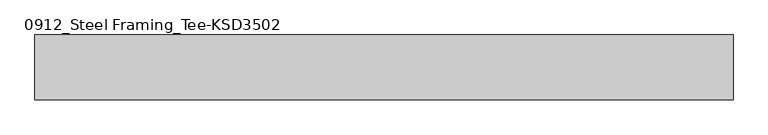
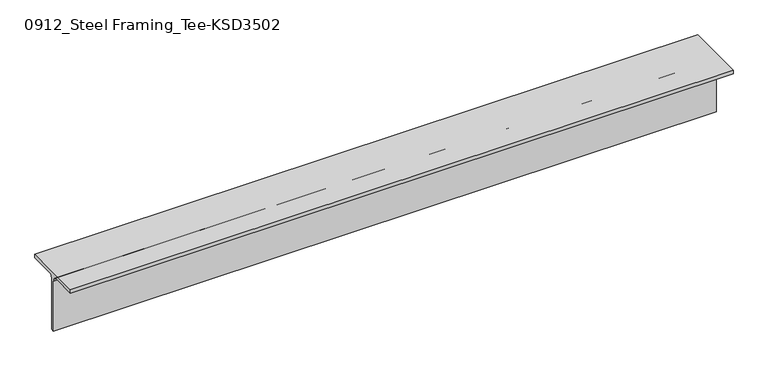
"""IFC4 building model written with IfcOpenShell, lengths in millimetres: member geometry, 0912_Steel Framing_Tee-KSD3502 : H_SB_ASB_CT-150x150x6.5x9."""

import ifcopenshell
import ifcopenshell.guid

model = None  # the IFC model being written
_history = None  # IfcOwnerHistory: only IFC2X3 demands one
_inside = {}  # id of a spatial element -> (the spatial element, [elements in it])
_under = {}  # id of a project, library or spatial element -> (it, [spatial elements below it])
_declared = {}  # id of a project -> (the project, [libraries it declares])
_typed = {}  # id of a type object -> (the type object, [elements of that type])
_made_of = {}  # id of a material, layer set ... -> (it, [elements and type objects made of it])


def new_model(schema):
    """Start an empty IFC model of exactly this schema.

    Asked for "IFC4X3", IfcOpenShell would pick the latest addendum, in which some entities
    have other attributes; the version numbers below select the first issue.
    IFC2X3 requires an IfcOwnerHistory on every rooted entity: one is made here for all.
    """
    global model, _history
    if schema == "IFC4X3":
        model = ifcopenshell.file(schema_version=(4, 3, 0, 0))
    else:
        model = ifcopenshell.file(schema=schema)
    _inside.clear()
    _under.clear()
    _declared.clear()
    _typed.clear()
    _made_of.clear()
    _history = None
    if model.schema == "IFC2X3":
        org = make("IfcOrganization", Name="unknown")
        user = make(
            "IfcPersonAndOrganization",
            ThePerson=make("IfcPerson", FamilyName="unknown"),
            TheOrganization=org,
        )
        app = make(
            "IfcApplication",
            ApplicationDeveloper=org,
            Version="unknown",
            ApplicationFullName="unknown",
            ApplicationIdentifier="unknown",
        )
        _history = make(
            "IfcOwnerHistory",
            OwningUser=user,
            OwningApplication=app,
            ChangeAction="ADDED",
            CreationDate=0,
        )
    return model


def make(cls, **values):
    """One entity of the class cls with the attributes given. An attribute that is None is left unset."""
    return model.create_entity(
        cls, **{name: value for name, value in values.items() if value is not None}
    )


def rooted(cls, **values):
    """An entity with a GlobalId (a new one), such as an element, a storey or a relation."""
    return make(cls, GlobalId=ifcopenshell.guid.new(), OwnerHistory=_history, **values)


def si_unit(unit_type, name, prefix=None):
    """IfcSIUnit, for example si_unit("LENGTHUNIT", "METRE", prefix="MILLI")."""
    return make("IfcSIUnit", UnitType=unit_type, Prefix=prefix, Name=name)


def assignment(units):
    """IfcUnitAssignment: the units of a project."""
    return None if units is None else make("IfcUnitAssignment", Units=units)


def point(xyz):
    """IfcCartesianPoint."""
    return None if xyz is None else make("IfcCartesianPoint", Coordinates=xyz)


def direction(xyz):
    """IfcDirection."""
    return None if xyz is None else make("IfcDirection", DirectionRatios=xyz)


def frame(location, z_axis=None, x_axis=None):
    """IfcAxis2Placement3D, a coordinate frame: its origin and axes. An axis left out is left unset."""
    return make(
        "IfcAxis2Placement3D",
        Location=point(location),
        Axis=direction(z_axis),
        RefDirection=direction(x_axis),
    )


def frame_2d(location, x_axis=None):
    """IfcAxis2Placement2D, a coordinate frame in the plane: its origin and x axis."""
    return make(
        "IfcAxis2Placement2D", Location=point(location), RefDirection=direction(x_axis)
    )


def origin():
    """The frame at (0, 0, 0) with its axes left unset."""
    return frame((0.0, 0.0, 0.0))


def place(relative_to, where):
    """IfcLocalPlacement: puts the frame where relative to a parent placement (None: the world)."""
    return make(
        "IfcLocalPlacement", PlacementRelTo=relative_to, RelativePlacement=where
    )


def context(
    kind, dimensions, precision=None, world=None, true_north=None, identifier=None
):
    """IfcGeometricRepresentationContext, for example the 3D "Model" context."""
    return make(
        "IfcGeometricRepresentationContext",
        ContextIdentifier=identifier,
        ContextType=kind,
        CoordinateSpaceDimension=dimensions,
        Precision=precision,
        WorldCoordinateSystem=world,
        TrueNorth=true_north,
    )


def project(units=None, contexts=None):
    """IfcProject with its units and contexts."""
    return rooted(
        "IfcProject",
        Name="project",
        RepresentationContexts=contexts,
        UnitsInContext=assignment(units),
    )


def spatial(cls, under=None, at=None, **own):
    """A site, building, storey or space (cls), placed at a placement, below another one or the project."""
    s = rooted(cls, ObjectPlacement=at, **own)
    if under is not None:
        _under.setdefault(under.id(), (under, []))[1].append(s)
    return s


def polyline(points):
    """IfcPolyline through the points."""
    return make("IfcPolyline", Points=[point(p) for p in points])


def circle_curve(where, radius):
    """IfcCircle in the frame where."""
    return make("IfcCircle", Position=where, Radius=radius)


def trimmed(basis, trim1, trim2, sense, master):
    """IfcTrimmedCurve: the piece of a basis curve between two trims."""
    return make(
        "IfcTrimmedCurve",
        BasisCurve=basis,
        Trim1=trim1,
        Trim2=trim2,
        SenseAgreement=sense,
        MasterRepresentation=master,
    )


def segment(curve, same_sense, transition):
    """IfcCompositeCurveSegment."""
    return make(
        "IfcCompositeCurveSegment",
        Transition=transition,
        SameSense=same_sense,
        ParentCurve=curve,
    )


def composite_curve(segments, self_intersect=None):
    """IfcCompositeCurve: segments joined end to end."""
    return make("IfcCompositeCurve", Segments=segments, SelfIntersect=self_intersect)


def outline(outer, holes=None, kind="AREA"):
    """IfcArbitraryClosedProfileDef: a profile drawn as a closed curve; with holes, ...WithVoids."""
    if holes is None:
        return make("IfcArbitraryClosedProfileDef", ProfileType=kind, OuterCurve=outer)
    return make(
        "IfcArbitraryProfileDefWithVoids",
        ProfileType=kind,
        OuterCurve=outer,
        InnerCurves=holes,
    )


def extrude(swept, where, along, depth):
    """IfcExtrudedAreaSolid: the profile swept, set in the frame where, extruded along a direction by depth."""
    return make(
        "IfcExtrudedAreaSolid",
        SweptArea=swept,
        Position=where,
        ExtrudedDirection=direction(along),
        Depth=depth,
    )


def shape(context_of_items, identifier, shape_type, items):
    """IfcShapeRepresentation: the items that make up one representation, for example the "Body"."""
    return make(
        "IfcShapeRepresentation",
        ContextOfItems=context_of_items,
        RepresentationIdentifier=identifier,
        RepresentationType=shape_type,
        Items=items,
    )


def source(mapping_origin, context_of_items, identifier, shape_type, items):
    """IfcRepresentationMap: a shape defined once, which mapped items show again and again."""
    return make(
        "IfcRepresentationMap",
        MappingOrigin=mapping_origin,
        MappedRepresentation=shape(context_of_items, identifier, shape_type, items),
    )


def transform(
    local_origin,
    x_axis=None,
    y_axis=None,
    z_axis=None,
    scale=None,
    scale2=None,
    scale3=None,
    uniform=True,
):
    """IfcCartesianTransformationOperator3D, or its non-uniform kind. x_axis, y_axis, z_axis: its Axis1, 2, 3."""
    if uniform:
        return make(
            "IfcCartesianTransformationOperator3D",
            Axis1=direction(x_axis),
            Axis2=direction(y_axis),
            LocalOrigin=point(local_origin),
            Scale=scale,
            Axis3=direction(z_axis),
        )
    return make(
        "IfcCartesianTransformationOperator3DnonUniform",
        Axis1=direction(x_axis),
        Axis2=direction(y_axis),
        LocalOrigin=point(local_origin),
        Scale=scale,
        Axis3=direction(z_axis),
        Scale2=scale2,
        Scale3=scale3,
    )


def mapped(mapping_source, mapping_target):
    """IfcMappedItem: shows the shape of a source again, moved by a transform."""
    return make(
        "IfcMappedItem", MappingSource=mapping_source, MappingTarget=mapping_target
    )


def made_of(thing, what):
    """Note that an element or type object is made of a material, layer set ...; save() writes the relation."""
    if what is not None:
        _made_of.setdefault(what.id(), (what, []))[1].append(thing)
    return thing


def element(
    cls,
    number,
    at=None,
    inside=None,
    cuts=None,
    type_object=None,
    material=None,
    context=None,
    identifier="Body",
    shape_type=None,
    held_by="IfcProductDefinitionShape",
    body=None,
    shapes=None,
    **own,
):
    """One element of the class cls, such as IfcWall. Its Tag is "e" and its number.

    at: its placement. inside: the storey or other place that contains it. cuts: it is an
    opening in that element (IfcRelVoidsElement). A single representation is given by context,
    identifier, shape_type and body (its items); several are given by shapes. held_by: the class
    of the entity that holds the representations. save() writes the other relations.
    """
    e = rooted(cls, Tag="e%d" % number, ObjectPlacement=at, **own)
    if body is not None:
        shapes = [shape(context, identifier, shape_type, body)]
    if shapes is not None:
        e.Representation = make(held_by, Representations=shapes)
    if inside is not None:
        _inside.setdefault(inside.id(), (inside, []))[1].append(e)
    if cuts is not None:
        rooted(
            "IfcRelVoidsElement", RelatingBuildingElement=cuts, RelatedOpeningElement=e
        )
    if type_object is not None:
        _typed.setdefault(type_object.id(), (type_object, []))[1].append(e)
    return made_of(e, material)


def aggregate(whole, parts):
    """IfcRelAggregates: a whole, such as a stair, and the parts it consists of."""
    return rooted("IfcRelAggregates", RelatingObject=whole, RelatedObjects=parts)


def save(model, path):
    """Write the relations noted so far, then the file.

    IfcRelAggregates (storeys below a building ...), IfcRelContainedInSpatialStructure (elements
    in a storey), IfcRelDefinesByType, IfcRelAssociatesMaterial and IfcRelDeclares: one each for
    every whole, place, type object, material and project.
    """
    for whole, parts in _under.values():
        aggregate(whole, parts)
    for where, things in _inside.values():
        rooted(
            "IfcRelContainedInSpatialStructure",
            RelatedElements=things,
            RelatingStructure=where,
        )
    for kind, things in _typed.values():
        rooted("IfcRelDefinesByType", RelatedObjects=things, RelatingType=kind)
    for what, things in _made_of.values():
        rooted("IfcRelAssociatesMaterial", RelatedObjects=things, RelatingMaterial=what)
    for by, libraries in _declared.values():
        rooted("IfcRelDeclares", RelatingContext=by, RelatedDefinitions=libraries)
    model.write(path)


def member_0912_steel_framing_tee_ksd3502_5d1e5f2d(model_context):
    return source(origin(), model_context, "Body", "SweptSolid", [
        extrude(outline(composite_curve([segment(polyline([(-75.0, 75.0), (75.0, 75.0), (75.0, 66.0), (16.25, 66.0)]), True, "CONTINUOUS"), segment(trimmed(circle_curve(frame_2d((16.25, 53.0)), 13.0), [point((16.25, 66.0))], [point((3.25, 53.0))], True, "CARTESIAN"), True, "CONTINUOUS"), segment(polyline([(3.25, 53.0), (3.25, -75.0), (-3.25, -75.0), (-3.25, 53.0)]), True, "CONTINUOUS"), segment(trimmed(circle_curve(frame_2d((-16.25, 53.0)), 13.0), [point((-3.25, 53.0))], [point((-16.25, 66.0))], True, "CARTESIAN"), True, "CONTINUOUS"), segment(polyline([(-16.25, 66.0), (-75.0, 66.0), (-75.0, 75.0)]), True, "CONTINUOUS")], self_intersect=False)), frame((-807.1, 0.0, 0.0), z_axis=(1.0, 0.0, 0.0), x_axis=(0.0, 1.0, 0.0)), (0.0, 0.0, 1.0), 1614.2),
    ])


if __name__ == "__main__":
    model = new_model("IFC4")
    model_context = context("Model", 3, world=origin())
    ifc_project = project(units=[si_unit("LENGTHUNIT", "METRE", prefix="MILLI")], contexts=[model_context])
    site = spatial("IfcSite", under=ifc_project)
    building = spatial("IfcBuilding", under=site)
    placement = place(None, origin())
    member_0912_steel_framing_tee_ksd3502_shape = member_0912_steel_framing_tee_ksd3502_5d1e5f2d(model_context)
    element("IfcMember", 1, ObjectType="0912_Steel Framing_Tee-KSD3502 : H_SB_ASB_CT-150x150x6.5x9", at=placement, inside=building, context=model_context, shape_type="MappedRepresentation", body=[
        mapped(member_0912_steel_framing_tee_ksd3502_shape, transform((0.0, 0.0, 0.0), x_axis=(1.0, 0.0, 0.0), y_axis=(0.0, 1.0, 0.0), z_axis=(0.0, 0.0, 1.0))),
    ])
    save(model, "model.ifc")

# Revit data of these elements
# Type "0912_Steel Framing_Tee-KSD3502 : H_SB_ASB_CT-150x150x6.5x9"
#   H_WM Code_1 = "S01AA003-00001 | Main Steel Structure Fabrication Work | Shelter/Building | Light Steel - Standard (30KG/M>Weight) | Material: (   )"
#   H_WM Code_2 = "S03AA029-00001 | Main Steel Structure Erection Work | Shelter/Building | Light Steel (30KG/M>Weight) | Material: (   )"
#   H_WM Code_3 = "S01AA010-00001 | Main Steel Structure Fabrication Work | Shelter/Building | Steel Painting/Coating | for Non-Fireproofed Steel Surface, Surface Preparation, Primer, Second & Final Coat | Material: (   )"
#   H_Q'ty Cal Type Tag = "SB-Q2"
#   Width = 15.0 cm
#   Web Thickness = 0.65 cm
#   Web Fillet = 1.3 cm
#   Section Area = 23.39 cm²
#   Perimeter = 0.60 m²/m
#   Nominal Weight = 18.40 kgf/m
#   Height = 15.0 cm
#   Flange Thickness = 0.9 cm
#   Centroid Vertical = 7.5 cm
#   Centroid Horizontal = 7.5 cm
#   Length [instance default] = 1.5000 m
#   Structural Material [instance default] = Steel, 45-345
#   Warping Constant = (empty or 0)
#   Torsional Moment of Inertia = 0
#   Section Name Key = ""
#   Plastic Modulus weak axis = 0
#   Plastic Modulus strong axis = 0
#   Moment of Inertia weak axis = 0
#   Moment of Inertia strong axis = 0
#   Elastic Modulus weak axis = 0
#   Elastic Modulus strong axis = 0
#   Bolt Spacing = 0
#   Assembly Code = ""
# Element 1 (IfcMember, "0912_Steel Framing_Tee-KSD3502 : H_SB_ASB_CT-150x150x6.5x9")
#   Structural Material = none
# Materials
#   "Steel, 45-345": class "Metal", colour RGB 189 187 185, transparency 0, Description = "Steel 345 MPa", Cost = 0
